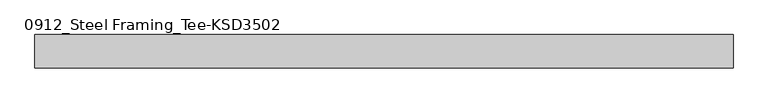
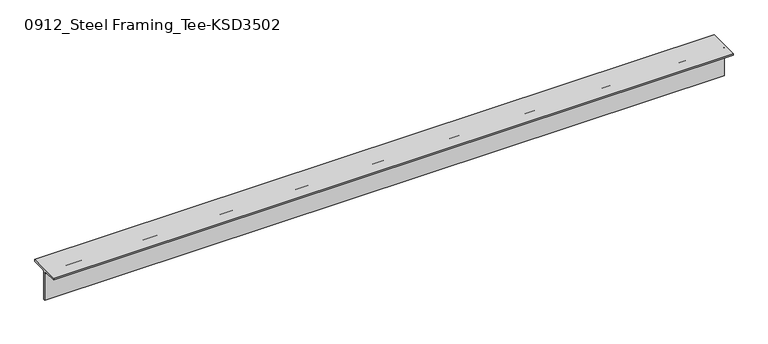
"""IFC4 building model written with IfcOpenShell, lengths in millimetres: member geometry, 0912_Steel Framing_Tee-KSD3502 : H_SB_ASB_CT-150x150x6.5x9."""

from ifc_helpers import new_model, si_unit, point, frame, frame_2d, origin, place, context, project, spatial, polyline, circle_curve, trimmed, segment, composite_curve, outline, extrude, source, transform, mapped, element, save


def member_0912_steel_framing_tee_ksd3502_53c68b3e(model_context):
    return source(origin(), model_context, "Body", "SweptSolid", [
        extrude(outline(composite_curve([segment(polyline([(-75.0, 75.0), (75.0, 75.0), (75.0, 66.0), (16.25, 66.0)]), True, "CONTINUOUS"), segment(trimmed(circle_curve(frame_2d((16.25, 53.0)), 13.0), [point((16.25, 66.0))], [point((3.25, 53.0))], True, "CARTESIAN"), True, "CONTINUOUS"), segment(polyline([(3.25, 53.0), (3.25, -75.0), (-3.25, -75.0), (-3.25, 53.0)]), True, "CONTINUOUS"), segment(trimmed(circle_curve(frame_2d((-16.25, 53.0)), 13.0), [point((-3.25, 53.0))], [point((-16.25, 66.0))], True, "CARTESIAN"), True, "CONTINUOUS"), segment(polyline([(-16.25, 66.0), (-75.0, 66.0), (-75.0, 75.0)]), True, "CONTINUOUS")], self_intersect=False)), frame((-1487.6, 0.0, 0.0), z_axis=(1.0, 0.0, 0.0), x_axis=(0.0, 1.0, 0.0)), (0.0, 0.0, 1.0), 3121.7),
    ])


if __name__ == "__main__":
    model = new_model("IFC4")
    model_context = context("Model", 3, world=origin())
    ifc_project = project(units=[si_unit("LENGTHUNIT", "METRE", prefix="MILLI")], contexts=[model_context])
    site = spatial("IfcSite", under=ifc_project)
    building = spatial("IfcBuilding", under=site)
    placement = place(None, origin())
    member_0912_steel_framing_tee_ksd3502_shape = member_0912_steel_framing_tee_ksd3502_53c68b3e(model_context)
    element("IfcMember", 1, ObjectType="0912_Steel Framing_Tee-KSD3502 : H_SB_ASB_CT-150x150x6.5x9", at=placement, inside=building, context=model_context, shape_type="MappedRepresentation", body=[
        mapped(member_0912_steel_framing_tee_ksd3502_shape, transform((0.0, 0.0, 0.0), x_axis=(1.0, 0.0, 0.0), y_axis=(0.0, 1.0, 0.0), z_axis=(0.0, 0.0, 1.0))),
    ])
    save(model, "model.ifc")

# Revit data of these elements
# Type "0912_Steel Framing_Tee-KSD3502 : H_SB_ASB_CT-150x150x6.5x9"
#   H_WM Code_1 = "S01AA003-00001 | Main Steel Structure Fabrication Work | Shelter/Building | Light Steel - Standard (30KG/M>Weight) | Material: (   )"
#   H_WM Code_2 = "S03AA029-00001 | Main Steel Structure Erection Work | Shelter/Building | Light Steel (30KG/M>Weight) | Material: (   )"
#   H_WM Code_3 = "S01AA010-00001 | Main Steel Structure Fabrication Work | Shelter/Building | Steel Painting/Coating | for Non-Fireproofed Steel Surface, Surface Preparation, Primer, Second & Final Coat | Material: (   )"
#   H_Q'ty Cal Type Tag = "SB-Q2"
#   Width = 15.0 cm
#   Web Thickness = 0.65 cm
#   Web Fillet = 1.3 cm
#   Section Area = 23.39 cm²
#   Perimeter = 0.60 m²/m
#   Nominal Weight = 18.40 kgf/m
#   Height = 15.0 cm
#   Flange Thickness = 0.9 cm
#   Centroid Vertical = 7.5 cm
#   Centroid Horizontal = 7.5 cm
#   Length [instance default] = 1.5000 m
#   Structural Material [instance default] = Steel, 45-345
#   Warping Constant = (empty or 0)
#   Torsional Moment of Inertia = 0
#   Section Name Key = ""
#   Plastic Modulus weak axis = 0
#   Plastic Modulus strong axis = 0
#   Moment of Inertia weak axis = 0
#   Moment of Inertia strong axis = 0
#   Elastic Modulus weak axis = 0
#   Elastic Modulus strong axis = 0
#   Bolt Spacing = 0
#   Assembly Code = ""
# Element 1 (IfcMember, "0912_Steel Framing_Tee-KSD3502 : H_SB_ASB_CT-150x150x6.5x9")
#   Structural Material = none
# Materials
#   "Steel, 45-345": class "Metal", colour RGB 189 187 185, transparency 0, Description = "Steel 345 MPa", Cost = 0
